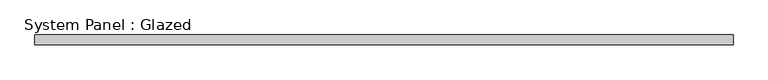
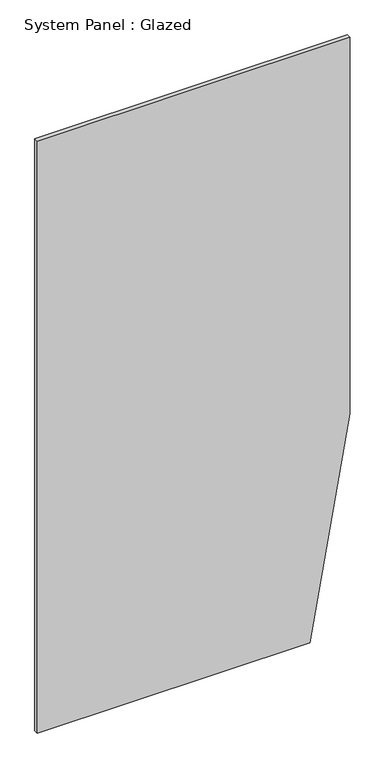
"""IFC4 building model written with IfcOpenShell, lengths in millimetres: plate geometry, System Panel : Glazed."""

import ifcopenshell
import ifcopenshell.guid

model = None  # the IFC model being written
_history = None  # IfcOwnerHistory: only IFC2X3 demands one
_inside = {}  # id of a spatial element -> (the spatial element, [elements in it])
_under = {}  # id of a project, library or spatial element -> (it, [spatial elements below it])
_declared = {}  # id of a project -> (the project, [libraries it declares])
_typed = {}  # id of a type object -> (the type object, [elements of that type])
_made_of = {}  # id of a material, layer set ... -> (it, [elements and type objects made of it])


def new_model(schema):
    """Start an empty IFC model of exactly this schema.

    Asked for "IFC4X3", IfcOpenShell would pick the latest addendum, in which some entities
    have other attributes; the version numbers below select the first issue.
    IFC2X3 requires an IfcOwnerHistory on every rooted entity: one is made here for all.
    """
    global model, _history
    if schema == "IFC4X3":
        model = ifcopenshell.file(schema_version=(4, 3, 0, 0))
    else:
        model = ifcopenshell.file(schema=schema)
    _inside.clear()
    _under.clear()
    _declared.clear()
    _typed.clear()
    _made_of.clear()
    _history = None
    if model.schema == "IFC2X3":
        org = make("IfcOrganization", Name="unknown")
        user = make(
            "IfcPersonAndOrganization",
            ThePerson=make("IfcPerson", FamilyName="unknown"),
            TheOrganization=org,
        )
        app = make(
            "IfcApplication",
            ApplicationDeveloper=org,
            Version="unknown",
            ApplicationFullName="unknown",
            ApplicationIdentifier="unknown",
        )
        _history = make(
            "IfcOwnerHistory",
            OwningUser=user,
            OwningApplication=app,
            ChangeAction="ADDED",
            CreationDate=0,
        )
    return model


def make(cls, **values):
    """One entity of the class cls with the attributes given. An attribute that is None is left unset."""
    return model.create_entity(
        cls, **{name: value for name, value in values.items() if value is not None}
    )


def rooted(cls, **values):
    """An entity with a GlobalId (a new one), such as an element, a storey or a relation."""
    return make(cls, GlobalId=ifcopenshell.guid.new(), OwnerHistory=_history, **values)


def si_unit(unit_type, name, prefix=None):
    """IfcSIUnit, for example si_unit("LENGTHUNIT", "METRE", prefix="MILLI")."""
    return make("IfcSIUnit", UnitType=unit_type, Prefix=prefix, Name=name)


def assignment(units):
    """IfcUnitAssignment: the units of a project."""
    return None if units is None else make("IfcUnitAssignment", Units=units)


def point(xyz):
    """IfcCartesianPoint."""
    return None if xyz is None else make("IfcCartesianPoint", Coordinates=xyz)


def direction(xyz):
    """IfcDirection."""
    return None if xyz is None else make("IfcDirection", DirectionRatios=xyz)


def frame(location, z_axis=None, x_axis=None):
    """IfcAxis2Placement3D, a coordinate frame: its origin and axes. An axis left out is left unset."""
    return make(
        "IfcAxis2Placement3D",
        Location=point(location),
        Axis=direction(z_axis),
        RefDirection=direction(x_axis),
    )


def origin():
    """The frame at (0, 0, 0) with its axes left unset."""
    return frame((0.0, 0.0, 0.0))


def place(relative_to, where):
    """IfcLocalPlacement: puts the frame where relative to a parent placement (None: the world)."""
    return make(
        "IfcLocalPlacement", PlacementRelTo=relative_to, RelativePlacement=where
    )


def context(
    kind, dimensions, precision=None, world=None, true_north=None, identifier=None
):
    """IfcGeometricRepresentationContext, for example the 3D "Model" context."""
    return make(
        "IfcGeometricRepresentationContext",
        ContextIdentifier=identifier,
        ContextType=kind,
        CoordinateSpaceDimension=dimensions,
        Precision=precision,
        WorldCoordinateSystem=world,
        TrueNorth=true_north,
    )


def project(units=None, contexts=None):
    """IfcProject with its units and contexts."""
    return rooted(
        "IfcProject",
        Name="project",
        RepresentationContexts=contexts,
        UnitsInContext=assignment(units),
    )


def spatial(cls, under=None, at=None, **own):
    """A site, building, storey or space (cls), placed at a placement, below another one or the project."""
    s = rooted(cls, ObjectPlacement=at, **own)
    if under is not None:
        _under.setdefault(under.id(), (under, []))[1].append(s)
    return s


def polyline(points):
    """IfcPolyline through the points."""
    return make("IfcPolyline", Points=[point(p) for p in points])


def outline(outer, holes=None, kind="AREA"):
    """IfcArbitraryClosedProfileDef: a profile drawn as a closed curve; with holes, ...WithVoids."""
    if holes is None:
        return make("IfcArbitraryClosedProfileDef", ProfileType=kind, OuterCurve=outer)
    return make(
        "IfcArbitraryProfileDefWithVoids",
        ProfileType=kind,
        OuterCurve=outer,
        InnerCurves=holes,
    )


def extrude(swept, where, along, depth):
    """IfcExtrudedAreaSolid: the profile swept, set in the frame where, extruded along a direction by depth."""
    return make(
        "IfcExtrudedAreaSolid",
        SweptArea=swept,
        Position=where,
        ExtrudedDirection=direction(along),
        Depth=depth,
    )


def shape(context_of_items, identifier, shape_type, items):
    """IfcShapeRepresentation: the items that make up one representation, for example the "Body"."""
    return make(
        "IfcShapeRepresentation",
        ContextOfItems=context_of_items,
        RepresentationIdentifier=identifier,
        RepresentationType=shape_type,
        Items=items,
    )


def source(mapping_origin, context_of_items, identifier, shape_type, items):
    """IfcRepresentationMap: a shape defined once, which mapped items show again and again."""
    return make(
        "IfcRepresentationMap",
        MappingOrigin=mapping_origin,
        MappedRepresentation=shape(context_of_items, identifier, shape_type, items),
    )


def transform(
    local_origin,
    x_axis=None,
    y_axis=None,
    z_axis=None,
    scale=None,
    scale2=None,
    scale3=None,
    uniform=True,
):
    """IfcCartesianTransformationOperator3D, or its non-uniform kind. x_axis, y_axis, z_axis: its Axis1, 2, 3."""
    if uniform:
        return make(
            "IfcCartesianTransformationOperator3D",
            Axis1=direction(x_axis),
            Axis2=direction(y_axis),
            LocalOrigin=point(local_origin),
            Scale=scale,
            Axis3=direction(z_axis),
        )
    return make(
        "IfcCartesianTransformationOperator3DnonUniform",
        Axis1=direction(x_axis),
        Axis2=direction(y_axis),
        LocalOrigin=point(local_origin),
        Scale=scale,
        Axis3=direction(z_axis),
        Scale2=scale2,
        Scale3=scale3,
    )


def mapped(mapping_source, mapping_target):
    """IfcMappedItem: shows the shape of a source again, moved by a transform."""
    return make(
        "IfcMappedItem", MappingSource=mapping_source, MappingTarget=mapping_target
    )


def made_of(thing, what):
    """Note that an element or type object is made of a material, layer set ...; save() writes the relation."""
    if what is not None:
        _made_of.setdefault(what.id(), (what, []))[1].append(thing)
    return thing


def element(
    cls,
    number,
    at=None,
    inside=None,
    cuts=None,
    type_object=None,
    material=None,
    context=None,
    identifier="Body",
    shape_type=None,
    held_by="IfcProductDefinitionShape",
    body=None,
    shapes=None,
    **own,
):
    """One element of the class cls, such as IfcWall. Its Tag is "e" and its number.

    at: its placement. inside: the storey or other place that contains it. cuts: it is an
    opening in that element (IfcRelVoidsElement). A single representation is given by context,
    identifier, shape_type and body (its items); several are given by shapes. held_by: the class
    of the entity that holds the representations. save() writes the other relations.
    """
    e = rooted(cls, Tag="e%d" % number, ObjectPlacement=at, **own)
    if body is not None:
        shapes = [shape(context, identifier, shape_type, body)]
    if shapes is not None:
        e.Representation = make(held_by, Representations=shapes)
    if inside is not None:
        _inside.setdefault(inside.id(), (inside, []))[1].append(e)
    if cuts is not None:
        rooted(
            "IfcRelVoidsElement", RelatingBuildingElement=cuts, RelatedOpeningElement=e
        )
    if type_object is not None:
        _typed.setdefault(type_object.id(), (type_object, []))[1].append(e)
    return made_of(e, material)


def aggregate(whole, parts):
    """IfcRelAggregates: a whole, such as a stair, and the parts it consists of."""
    return rooted("IfcRelAggregates", RelatingObject=whole, RelatedObjects=parts)


def save(model, path):
    """Write the relations noted so far, then the file.

    IfcRelAggregates (storeys below a building ...), IfcRelContainedInSpatialStructure (elements
    in a storey), IfcRelDefinesByType, IfcRelAssociatesMaterial and IfcRelDeclares: one each for
    every whole, place, type object, material and project.
    """
    for whole, parts in _under.values():
        aggregate(whole, parts)
    for where, things in _inside.values():
        rooted(
            "IfcRelContainedInSpatialStructure",
            RelatedElements=things,
            RelatingStructure=where,
        )
    for kind, things in _typed.values():
        rooted("IfcRelDefinesByType", RelatedObjects=things, RelatingType=kind)
    for what, things in _made_of.values():
        rooted("IfcRelAssociatesMaterial", RelatedObjects=things, RelatingMaterial=what)
    for by, libraries in _declared.values():
        rooted("IfcRelDeclares", RelatingContext=by, RelatedDefinitions=libraries)
    model.write(path)


def system_panel_glazed_87679f4c(model_context):
    return source(origin(), model_context, "Body", "SweptSolid", [
        extrude(outline(polyline([(0.0, -914.4), (0.0, 680.3834794), (1332.2432262, 914.4), (3657.6, 914.4), (3657.6, -914.4), (0.0, -914.4)])), frame((0.0, -44.45, 0.0), z_axis=(0.0, 1.0, 0.0), x_axis=(0.0, 0.0, 1.0)), (0.0, 0.0, 1.0), 25.4),
    ])


if __name__ == "__main__":
    model = new_model("IFC4")
    model_context = context("Model", 3, world=origin())
    ifc_project = project(units=[si_unit("LENGTHUNIT", "METRE", prefix="MILLI")], contexts=[model_context])
    site = spatial("IfcSite", under=ifc_project)
    building = spatial("IfcBuilding", under=site)
    placement = place(None, origin())
    system_panel_glazed_shape = system_panel_glazed_87679f4c(model_context)
    element("IfcPlate", 1, ObjectType="System Panel : Glazed", at=placement, inside=building, context=model_context, shape_type="MappedRepresentation", body=[
        mapped(system_panel_glazed_shape, transform((0.0, 0.0, 0.0), x_axis=(1.0, 0.0, 0.0), y_axis=(0.0, 1.0, 0.0), z_axis=(0.0, 0.0, 1.0))),
    ])
    save(model, "model.ifc")

# Revit data of these elements
# Type "System Panel : Glazed"
#   Construction Type Id = "GSP4R"
#   Analytic Construction = "1/8 in Pilkington single glazing"
#   Visual Light Transmittance = 0.9
#   Solar Heat Gain Coefficient = 0.86
#   Heat Transfer Coefficient (U) = 1.18115 BTU/(h·ft²·°F)
#   Define Thermal Properties by = 1
# Element 1 (IfcPlate, "System Panel : Glazed")
#   Materials on its faces: "Glass"
# Materials
#   "Glass": class "Glass", colour RGB 0 128 192, transparency 0.75, Description = "Soda Lime Glass", Cost = 0
